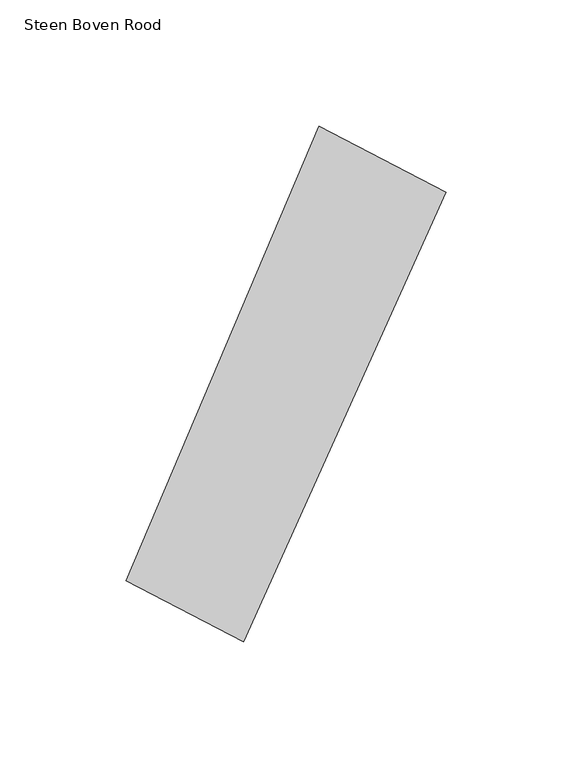
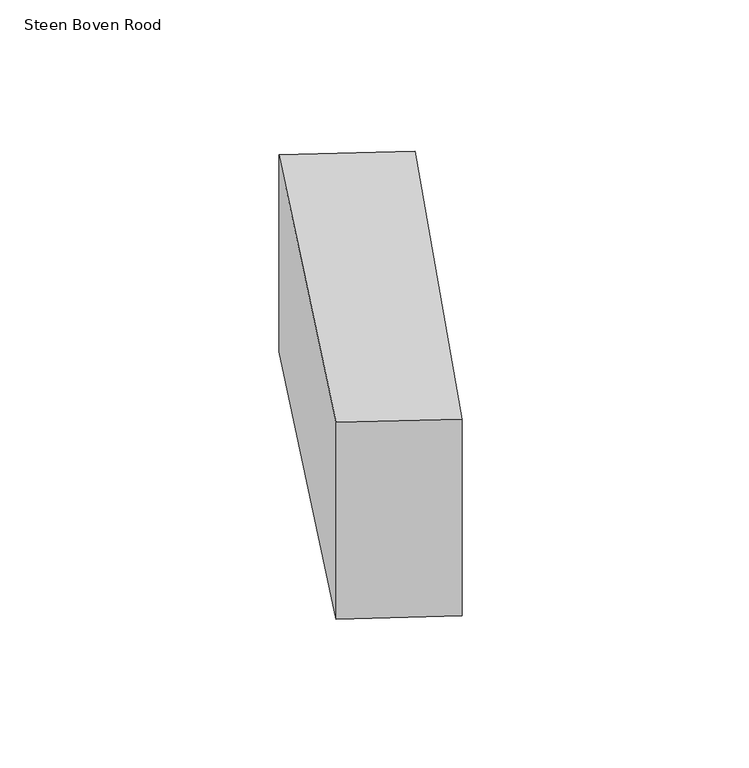
"""IFC4 building model written with IfcOpenShell, lengths in millimetres: proxy geometry, 00_GMA_steen_versie_4 : Steen Boven Rood."""

from ifc_helpers import new_model, si_unit, origin, origin_with_axes, place, context, project, spatial, polyline, outline, extrude, source, transform, mapped, element, save


def steen_boven_rood_581125f1(model_context):
    return source(origin(), model_context, "Body", "SweptSolid", [
        extrude(outline(polyline([(142.2710112, 162.2083541), (62.0148263, -15.8493548), (15.5681365, 8.2629874), (91.9807854, 188.323566), (142.2710112, 162.2083541)])), origin_with_axes(), (0.0, 0.0, 1.0), 100.0),
    ])


if __name__ == "__main__":
    model = new_model("IFC4")
    model_context = context("Model", 3, world=origin())
    ifc_project = project(units=[si_unit("LENGTHUNIT", "METRE", prefix="MILLI")], contexts=[model_context])
    site = spatial("IfcSite", under=ifc_project)
    building = spatial("IfcBuilding", under=site)
    placement = place(None, origin())
    steen_boven_rood_shape = steen_boven_rood_581125f1(model_context)
    element("IfcBuildingElementProxy", 1, Name="00_GMA_steen_versie_4 : Steen Boven Rood", ObjectType="00_GMA_steen_versie_4 : Steen Boven Rood", at=placement, inside=building, context=model_context, shape_type="MappedRepresentation", body=[
        mapped(steen_boven_rood_shape, transform((0.0, 0.0, 0.0), x_axis=(1.0, 0.0, 0.0), y_axis=(0.0, 1.0, 0.0), z_axis=(0.0, 0.0, 1.0))),
    ])
    save(model, "model.ifc")

# Revit data of these elements
# Type "00_GMA_steen_versie_4 : Steen Boven Rood"
#   StootVoegHalfBoven [instance default] = 5 mm
#   StootVoegHalf [instance default] = 5 mm
#   StootVoegBreedteOnder = 10 mm
#   StootVoegBreedteBoven = 10 mm
#   Steendikte = 100 mm
#   LintVoegOnderHalf = 5 mm
#   LintVoegOnder = 10 mm
#   LintVoegBovenHalf = 0 mm
#   LintVoegBoven = 0 mm
#   materiaal = 21_steen_rood
#   MateriaalVoeg = none
#   Default Elevation = 0
# Element 1 (IfcBuildingElementProxy, "00_GMA_steen_versie_4 : Steen Boven Rood")
#   Materials on its faces: "21_steen_rood"
# Materials
#   "21_steen_rood": class "Unassigned", colour RGB 213 111 43, transparency 0, Cost = 0
